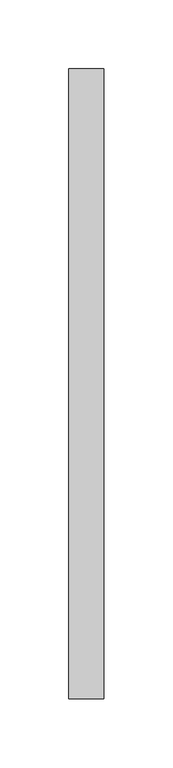
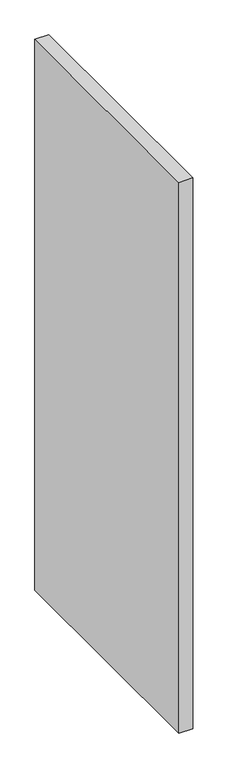
"""IFC4 building model written with IfcOpenShell, lengths in millimetres: proxy geometry."""

from ifc_helpers import new_model, si_unit, frame, origin, place, context, project, spatial, polyline, outline, extrude, source, transform, mapped, element, save


def specialty_equipment_2d138f7b(model_context):
    return source(origin(), model_context, "Body", "SweptSolid", [
        extrude(outline(polyline([(12.7, -198.4375), (12.7, -655.6375), (-12.7, -655.6375), (-12.7, -198.4375), (12.7, -198.4375)])), frame((0.0, 0.0, 355.6), z_axis=(0.0, 0.0, 1.0), x_axis=(1.0, 0.0, 0.0)), (0.0, 0.0, 1.0), 1066.8),
    ])


if __name__ == "__main__":
    model = new_model("IFC4")
    model_context = context("Model", 3, world=origin())
    ifc_project = project(units=[si_unit("LENGTHUNIT", "METRE", prefix="MILLI")], contexts=[model_context])
    site = spatial("IfcSite", under=ifc_project)
    building = spatial("IfcBuilding", under=site)
    placement = place(None, origin())
    specialty_equipment_shape = specialty_equipment_2d138f7b(model_context)
    element("IfcBuildingElementProxy", 1, Name="Urinal Screen-3D w Urinal : 36\" O.C.", ObjectType="Urinal Screen-3D w Urinal : 36\" O.C.", at=placement, inside=building, context=model_context, shape_type="MappedRepresentation", body=[
        mapped(specialty_equipment_shape, transform((0.0, 0.0, 0.0), x_axis=(1.0, 0.0, 0.0), y_axis=(0.0, 1.0, 0.0), z_axis=(0.0, 0.0, 1.0))),
    ])
    save(model, "model.ifc")

# Revit data of these elements
# Type "Urinal Screen-3D w Urinal : 36\" O.C."
#   Assembly Code = "C1030100"
#   O.C. = 3' - 0"
#   Depth = 1' - 6"
#   Toilet Partition Material = Toilet Partition
#   Default Elevation = 0
# Element 1 (IfcBuildingElementProxy, "Urinal Screen-3D w Urinal : 36\" O.C.")
#   Materials on its faces: "Toilet Partition"
# Materials
#   "Toilet Partition": class "Unassigned", colour RGB 0 181 188, transparency 0
